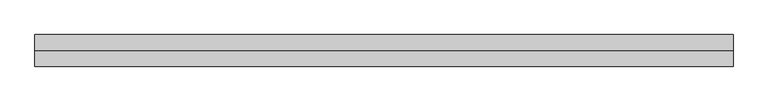
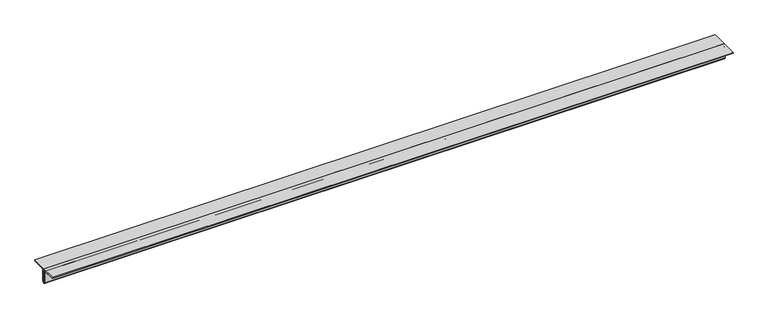
"""IFC4 building model written with IfcOpenShell, lengths in millimetres: member geometry, 0123_Steel Framing_2Ls-KSD3502 : H_SB_AR_S03_2Ls-130x130x12_HBR4."""

from ifc_helpers import new_model, si_unit, point, frame, frame_2d, origin, place, context, project, spatial, polyline, circle_curve, trimmed, segment, composite_curve, outline, extrude, source, transform, mapped, element, save


def member_1fece13f(model_context):
    return source(origin(), model_context, "Body", "SweptSolid", [
        extrude(outline(composite_curve([segment(polyline([(0.0, 36.4), (130.0, 36.4)]), True, "CONTINUOUS"), segment(trimmed(circle_curve(frame_2d((118.0, 36.4)), 12.0), [point((130.0, 36.4))], [point((118.0, 24.4))], False, "CARTESIAN"), True, "CONTINUOUS"), segment(polyline([(118.0, 24.4), (24.0, 24.4)]), True, "CONTINUOUS"), segment(trimmed(circle_curve(frame_2d((24.0, 12.4)), 12.0), [point((24.0, 24.4))], [point((12.0, 12.4))], True, "CARTESIAN"), True, "CONTINUOUS"), segment(polyline([(12.0, 12.4), (12.0, -81.6)]), True, "CONTINUOUS"), segment(trimmed(circle_curve(frame_2d((0.0, -81.6)), 12.0), [point((12.0, -81.6))], [point((0.0, -93.6))], False, "CARTESIAN"), True, "CONTINUOUS"), segment(polyline([(0.0, -93.6), (0.0, 36.4)]), True, "CONTINUOUS")], self_intersect=False)), frame((-2932.893323, 0.0, 0.0), z_axis=(1.0, 0.0, 0.0), x_axis=(0.0, 1.0, 0.0)), (0.0, 0.0, 1.0), 5733.5453123),
        extrude(outline(composite_curve([segment(polyline([(0.0, 36.4), (0.0, -93.6)]), True, "CONTINUOUS"), segment(trimmed(circle_curve(frame_2d((0.0, -81.6)), 12.0), [point((0.0, -93.6))], [point((-12.0, -81.6))], False, "CARTESIAN"), True, "CONTINUOUS"), segment(polyline([(-12.0, -81.6), (-12.0, 12.4)]), True, "CONTINUOUS"), segment(trimmed(circle_curve(frame_2d((-24.0, 12.4)), 12.0), [point((-12.0, 12.4))], [point((-24.0, 24.4))], True, "CARTESIAN"), True, "CONTINUOUS"), segment(polyline([(-24.0, 24.4), (-118.0, 24.4)]), True, "CONTINUOUS"), segment(trimmed(circle_curve(frame_2d((-118.0, 36.4)), 12.0), [point((-118.0, 24.4))], [point((-130.0, 36.4))], False, "CARTESIAN"), True, "CONTINUOUS"), segment(polyline([(-130.0, 36.4), (0.0, 36.4)]), True, "CONTINUOUS")], self_intersect=False)), frame((-2932.893323, 0.0, 0.0), z_axis=(1.0, 0.0, 0.0), x_axis=(0.0, 1.0, 0.0)), (0.0, 0.0, 1.0), 5733.5453123),
    ])


if __name__ == "__main__":
    model = new_model("IFC4")
    model_context = context("Model", 3, world=origin())
    ifc_project = project(units=[si_unit("LENGTHUNIT", "METRE", prefix="MILLI")], contexts=[model_context])
    site = spatial("IfcSite", under=ifc_project)
    building = spatial("IfcBuilding", under=site)
    placement = place(None, origin())
    member_shape = member_1fece13f(model_context)
    element("IfcMember", 1, ObjectType="0123_Steel Framing_2Ls-KSD3502 : H_SB_AR_S03_2Ls-130x130x12_HBR4", at=placement, inside=building, context=model_context, shape_type="MappedRepresentation", body=[
        mapped(member_shape, transform((0.0, 0.0, 0.0), x_axis=(1.0, 0.0, 0.0), y_axis=(0.0, 1.0, 0.0), z_axis=(0.0, 0.0, 1.0))),
    ])
    save(model, "model.ifc")

# Revit data of these elements
# Type "0123_Steel Framing_2Ls-KSD3502 : H_SB_AR_S03_2Ls-130x130x12_HBR4"
#   Type Mark = "HBR4"
#   Assembly Code = "B10"
#   Legs = "SLBB"
#   W = 8.97
#   Perimeter = 1.04 m²/m
#   Nominal Weight = 46.80 kgf/m
#   Length [instance default] = 1000 mm
#   Space = 0 mm
#   b = 130 mm
#   d = 130 mm
#   t = 12 mm
#   y = 36.4 mm
#   A = 0.005952 m²
#   Structural Material [instance default] = Steel ASTM A36
# Element 1 (IfcMember, "0123_Steel Framing_2Ls-KSD3502 : H_SB_AR_S03_2Ls-130x130x12_HBR4")
#   Materials on its faces: "Steel ASTM A36"
# Materials
#   "Steel ASTM A36": class "Metal", colour RGB 199 199 199, transparency 0, Description = "Structural steel, ASTM A36 Grade B, mill finish", Cost = 0
